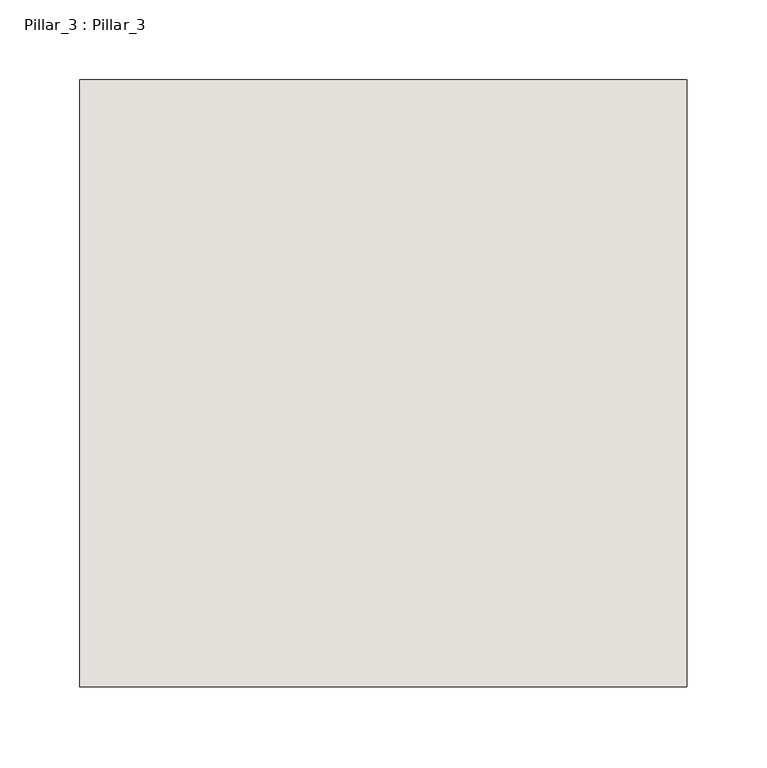
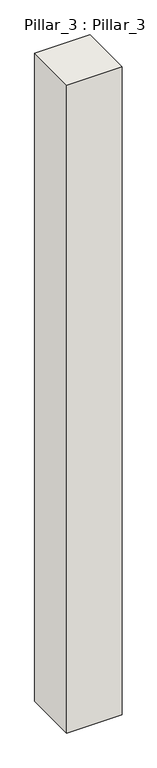
"""IFC4 building model written with IfcOpenShell, lengths in millimetres: wall geometry, Pillar_3 : Pillar_3."""

from ifc_helpers import new_model, si_unit, origin, origin_with_axes, place, context, project, spatial, polyline, outline, extrude, source, transform, mapped, element, save


def pillar_3_pillar_3_bef34371(model_context):
    return source(origin(), model_context, "Body", "SweptSolid", [
        extrude(outline(polyline([(240.0, 7510.0), (-140.0, 7510.0), (-140.0, 7890.0), (240.0, 7890.0), (240.0, 7510.0)])), origin_with_axes(), (0.0, 0.0, 1.0), 4700.0),
    ])


if __name__ == "__main__":
    model = new_model("IFC4")
    model_context = context("Model", 3, world=origin())
    ifc_project = project(units=[si_unit("LENGTHUNIT", "METRE", prefix="MILLI")], contexts=[model_context])
    site = spatial("IfcSite", under=ifc_project)
    building = spatial("IfcBuilding", under=site)
    placement = place(None, origin())
    pillar_3_pillar_3_shape = pillar_3_pillar_3_bef34371(model_context)
    element("IfcWall", 1, ObjectType="Pillar_3 : Pillar_3", at=placement, inside=building, context=model_context, shape_type="MappedRepresentation", body=[
        mapped(pillar_3_pillar_3_shape, transform((0.0, 0.0, 0.0), x_axis=(1.0, 0.0, 0.0), y_axis=(0.0, 1.0, 0.0), z_axis=(0.0, 0.0, 1.0))),
    ])
    save(model, "model.ifc")

# Revit data of these elements
# Type "Pillar_3 : Pillar_3"
#   NameOverride = "Pillar_3"
# Element 1 (IfcWall, "Pillar_3 : Pillar_3")
#   Materials on its faces: "IfcSurfaceStyle #33"
# Materials
#   "IfcSurfaceStyle #33": class "Unassigned", colour RGB 214 214 214, transparency 0
